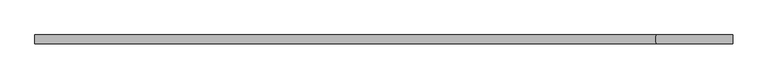
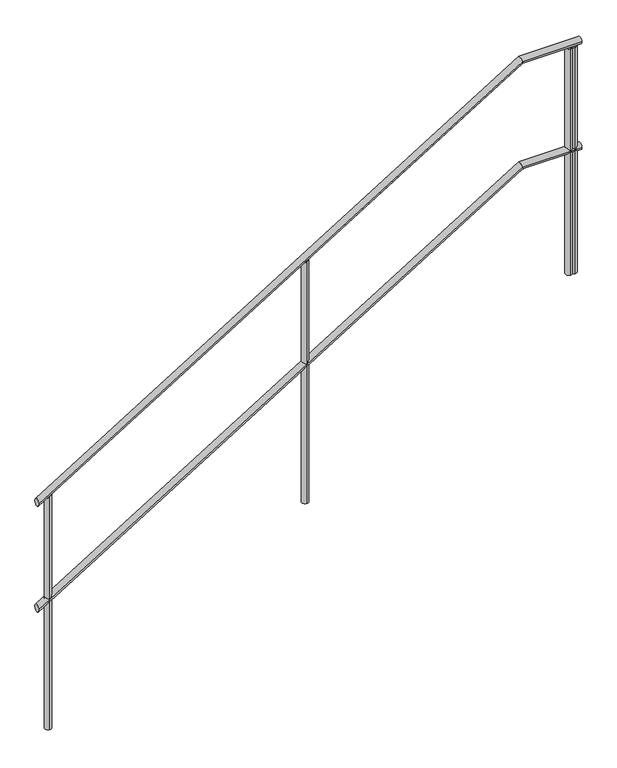
"""IFC4 building model written with IfcOpenShell, lengths in millimetres: railing geometry."""

from ifc_helpers import new_model, si_unit, point, frame, frame_2d, origin, place, context, project, spatial, circle_curve, ellipse_curve, trimmed, segment, composite_curve, outline, extrude, source, transform, mapped, element, save
from ifc_brep_helpers import plane_surface, cylinder_surface, advanced_brep


def railing_e17628cd(model_context):
    return source(origin(), model_context, "Body", "SolidModel", [
        advanced_brep(
        [(3184.0, -1867.9791411, -450.9609787), (3184.0, -1837.9791411, -450.9609787), (5348.2567855, -1837.9791411, 885.0), (5348.2567855, -1867.9791411, 885.0), (5614.0, -1867.9791411, 885.0), (5614.0, -1837.9791411, 885.0)],
        [
            (0, 1, ellipse_curve(frame((3184.0, -1852.9791411, -450.9609787), z_axis=(-1.0, 0.0, 0.0), x_axis=(0.0, 0.0, -1.0)), 17.6276454, 15.0)),
            (1, 0, ellipse_curve(frame((3184.0, -1852.9791411, -450.9609787), z_axis=(-1.0, 0.0, 0.0), x_axis=(0.0, 0.0, -1.0)), 17.6276454, 15.0)),
            (1, 2),
            (2, 3, ellipse_curve(frame((5348.2567855, -1852.9791411, 885.0), z_axis=(-0.9620125025549408, 0.0, -0.2730053935877092), x_axis=(0.2730053935877087, 0.0, -0.962012502554941)), 15.5923129, 15.0)),
            (3, 0),
            (3, 2, ellipse_curve(frame((5348.2567855, -1852.9791411, 885.0), z_axis=(-0.9620125025549408, 0.0, -0.2730053935877092), x_axis=(0.2730053935877087, 0.0, -0.962012502554941)), 15.5923129, 15.0)),
            (4, 5, circle_curve(frame((5614.0, -1852.9791411, 885.0), z_axis=(1.0, 0.0, 0.0), x_axis=(0.0, 1.0, 0.0)), 15.0)),
            (5, 4, circle_curve(frame((5614.0, -1852.9791411, 885.0), z_axis=(1.0, 0.0, 0.0), x_axis=(0.0, 1.0, 0.0)), 15.0)),
            (2, 5),
            (4, 3),
        ],
        [
            plane_surface(frame((3184.0, -1852.9791411, -433.3333333), z_axis=(-1.0, 0.0, 0.0), x_axis=(0.0, 1.0, 0.0))),
            cylinder_surface(frame((3191.8790381, -1852.9791411, -446.097375), z_axis=(-0.8509361101440399, 0.0, -0.5252692037926174), x_axis=(0.0, 1.0, 0.0)), 15.0),
            plane_surface(frame((5614.0, -1852.9791411, 900.0), z_axis=(1.0, 0.0, 0.0), x_axis=(0.0, 1.0, 0.0))),
            cylinder_surface(frame((5344.0, -1852.9791411, 885.0), z_axis=(-1.0, 0.0, 0.0), x_axis=(0.0, 1.0, 0.0)), 15.0),
        ],
        [
            (0, [[1, 2]]),
            (1, [[-2, 3, 4, 5]]),
            (1, [[-1, -5, 6, -3]]),
            (2, [[7, 8]]),
            (3, [[-4, 9, -7, 10]]),
            (3, [[-6, -10, -8, -9]]),
        ],
    ),
        advanced_brep(
        [(3184.0, -1867.9791411, 49.0390213), (3184.0, -1837.9791411, 49.0390213), (5348.2567855, -1837.9791411, 1385.0), (5348.2567855, -1867.9791411, 1385.0), (5614.0, -1867.9791411, 1385.0), (5614.0, -1837.9791411, 1385.0)],
        [
            (0, 1, ellipse_curve(frame((3184.0, -1852.9791411, 49.0390213), z_axis=(-1.0, 0.0, 0.0), x_axis=(0.0, 0.0, -1.0)), 17.6276454, 15.0)),
            (1, 0, ellipse_curve(frame((3184.0, -1852.9791411, 49.0390213), z_axis=(-1.0, 0.0, 0.0), x_axis=(0.0, 0.0, -1.0)), 17.6276454, 15.0)),
            (1, 2),
            (2, 3, ellipse_curve(frame((5348.2567855, -1852.9791411, 1385.0), z_axis=(-0.9620125025549408, 0.0, -0.2730053935877092), x_axis=(0.2730053935877087, 0.0, -0.962012502554941)), 15.5923129, 15.0)),
            (3, 0),
            (3, 2, ellipse_curve(frame((5348.2567855, -1852.9791411, 1385.0), z_axis=(-0.9620125025549408, 0.0, -0.2730053935877092), x_axis=(0.2730053935877087, 0.0, -0.962012502554941)), 15.5923129, 15.0)),
            (4, 5, circle_curve(frame((5614.0, -1852.9791411, 1385.0), z_axis=(1.0, 0.0, 0.0), x_axis=(0.0, 1.0, 0.0)), 15.0)),
            (5, 4, circle_curve(frame((5614.0, -1852.9791411, 1385.0), z_axis=(1.0, 0.0, 0.0), x_axis=(0.0, 1.0, 0.0)), 15.0)),
            (2, 5),
            (4, 3),
        ],
        [
            plane_surface(frame((3184.0, -1852.9791411, 66.6666667), z_axis=(-1.0, 0.0, 0.0), x_axis=(0.0, 1.0, 0.0))),
            cylinder_surface(frame((3191.8790381, -1852.9791411, 53.902625), z_axis=(-0.8509361101440399, 0.0, -0.5252692037926174), x_axis=(0.0, 1.0, 0.0)), 15.0),
            plane_surface(frame((5614.0, -1852.9791411, 1400.0), z_axis=(1.0, 0.0, 0.0), x_axis=(0.0, 1.0, 0.0))),
            cylinder_surface(frame((5344.0, -1852.9791411, 1385.0), z_axis=(-1.0, 0.0, 0.0), x_axis=(0.0, 1.0, 0.0)), 15.0),
        ],
        [
            (0, [[1, 2]]),
            (1, [[-2, 3, 4, 5]]),
            (1, [[-1, -5, 6, -3]]),
            (2, [[7, 8]]),
            (3, [[-4, 9, -7, 10]]),
            (3, [[-6, -10, -8, -9]]),
        ],
    ),
        extrude(outline(composite_curve([segment(trimmed(circle_curve(frame_2d((5584.0, -1852.9791411)), 15.0), [point((5584.0, -1867.9791411))], [point((5584.0, -1837.9791411))], False, "CARTESIAN"), True, "CONTINUOUS"), segment(trimmed(circle_curve(frame_2d((5584.0, -1852.9791411)), 15.0), [point((5584.0, -1837.9791411))], [point((5584.0, -1867.9791411))], False, "CARTESIAN"), True, "CONTINUOUS")], self_intersect=False)), frame((0.0, 0.0, 300.0), z_axis=(0.0, 0.0, 1.0), x_axis=(1.0, 0.0, 0.0)), (0.0, 0.0, 1.0), 1070.0),
        advanced_brep(
        [(4384.0, -1837.9791411, 777.4074074), (4384.0, -1867.9791411, 777.4074074), (4384.0, -1867.9791411, -366.6666667), (4384.0, -1837.9791411, -366.6666667)],
        [
            (0, 1, ellipse_curve(frame((4384.0, -1852.9791411, 777.4074074), z_axis=(0.5252692037926167, 0.0, -0.8509361101440406), x_axis=(0.8509361101440406, 0.0, 0.5252692037926162)), 17.6276454, 15.0)),
            (1, 2),
            (2, 3, circle_curve(frame((4384.0, -1852.9791411, -366.6666667), z_axis=(0.0, 0.0, 1.0), x_axis=(0.0, -1.0, 0.0)), 15.0)),
            (3, 0),
            (3, 2, circle_curve(frame((4384.0, -1852.9791411, -366.6666667), z_axis=(0.0, 0.0, 1.0), x_axis=(0.0, -1.0, 0.0)), 15.0)),
            (1, 0, ellipse_curve(frame((4384.0, -1852.9791411, 777.4074074), z_axis=(0.5252692037926167, 0.0, -0.8509361101440406), x_axis=(0.8509361101440406, 0.0, 0.5252692037926162)), 17.6276454, 15.0)),
        ],
        [
            cylinder_surface(frame((4384.0, -1852.9791411, -466.6666667), z_axis=(0.0, 0.0, 1.0), x_axis=(0.0, -1.0, 0.0)), 15.0),
            plane_surface(frame((4409.0, -1877.9791411, 792.8395062), z_axis=(-0.5252692037926167, 0.0, 0.8509361101440406), x_axis=(0.0, 1.0, 0.0))),
            plane_surface(frame((4359.0, -1877.9791411, -366.6666667), z_axis=(0.0, 0.0, -1.0), x_axis=(0.0, 1.0, 0.0))),
        ],
        [
            (0, [[1, 2, 3, 4]]),
            (0, [[5, -2, 6, -4]]),
            (1, [[-6, -1]]),
            (2, [[-5, -3]]),
        ],
    ),
        extrude(outline(composite_curve([segment(trimmed(circle_curve(frame_2d((5564.0, -1852.9791411)), 15.0), [point((5564.0, -1867.9791411))], [point((5564.0, -1837.9791411))], False, "CARTESIAN"), True, "CONTINUOUS"), segment(trimmed(circle_curve(frame_2d((5564.0, -1852.9791411)), 15.0), [point((5564.0, -1837.9791411))], [point((5564.0, -1867.9791411))], False, "CARTESIAN"), True, "CONTINUOUS")], self_intersect=False)), frame((0.0, 0.0, 300.0), z_axis=(0.0, 0.0, 1.0), x_axis=(1.0, 0.0, 0.0)), (0.0, 0.0, 1.0), 1070.0),
        advanced_brep(
        [(3234.0, -1837.9791411, 67.5308642), (3234.0, -1867.9791411, 67.5308642), (3234.0, -1867.9791411, -1033.3333333), (3234.0, -1837.9791411, -1033.3333333)],
        [
            (0, 1, ellipse_curve(frame((3234.0, -1852.9791411, 67.5308642), z_axis=(0.5252692037926167, 0.0, -0.8509361101440406), x_axis=(0.8509361101440406, 0.0, 0.5252692037926162)), 17.6276454, 15.0)),
            (1, 2),
            (2, 3, circle_curve(frame((3234.0, -1852.9791411, -1033.3333333), z_axis=(0.0, 0.0, 1.0), x_axis=(0.0, -1.0, 0.0)), 15.0)),
            (3, 0),
            (3, 2, circle_curve(frame((3234.0, -1852.9791411, -1033.3333333), z_axis=(0.0, 0.0, 1.0), x_axis=(0.0, -1.0, 0.0)), 15.0)),
            (1, 0, ellipse_curve(frame((3234.0, -1852.9791411, 67.5308642), z_axis=(0.5252692037926167, 0.0, -0.8509361101440406), x_axis=(0.8509361101440406, 0.0, 0.5252692037926162)), 17.6276454, 15.0)),
        ],
        [
            cylinder_surface(frame((3234.0, -1852.9791411, -1133.3333333), z_axis=(0.0, 0.0, 1.0), x_axis=(0.0, -1.0, 0.0)), 15.0),
            plane_surface(frame((3259.0, -1877.9791411, 82.962963), z_axis=(-0.5252692037926167, 0.0, 0.8509361101440406), x_axis=(0.0, 1.0, 0.0))),
            plane_surface(frame((3209.0, -1877.9791411, -1033.3333333), z_axis=(0.0, 0.0, -1.0), x_axis=(0.0, 1.0, 0.0))),
        ],
        [
            (0, [[1, 2, 3, 4]]),
            (0, [[5, -2, 6, -4]]),
            (1, [[-6, -1]]),
            (2, [[-5, -3]]),
        ],
    ),
    ])


if __name__ == "__main__":
    model = new_model("IFC4")
    model_context = context("Model", 3, world=origin())
    ifc_project = project(units=[si_unit("LENGTHUNIT", "METRE", prefix="MILLI")], contexts=[model_context])
    site = spatial("IfcSite", under=ifc_project)
    building = spatial("IfcBuilding", under=site)
    placement = place(None, origin())
    railing_shape = railing_e17628cd(model_context)
    element("IfcRailing", 1, at=placement, inside=building, context=model_context, shape_type="MappedRepresentation", body=[
        mapped(railing_shape, transform((0.0, 0.0, 0.0), x_axis=(1.0, 0.0, 0.0), y_axis=(0.0, 1.0, 0.0), z_axis=(0.0, 0.0, 1.0))),
    ])
    save(model, "model.ifc")
